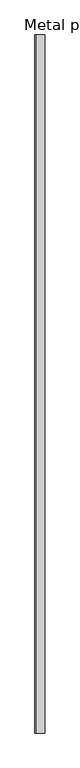
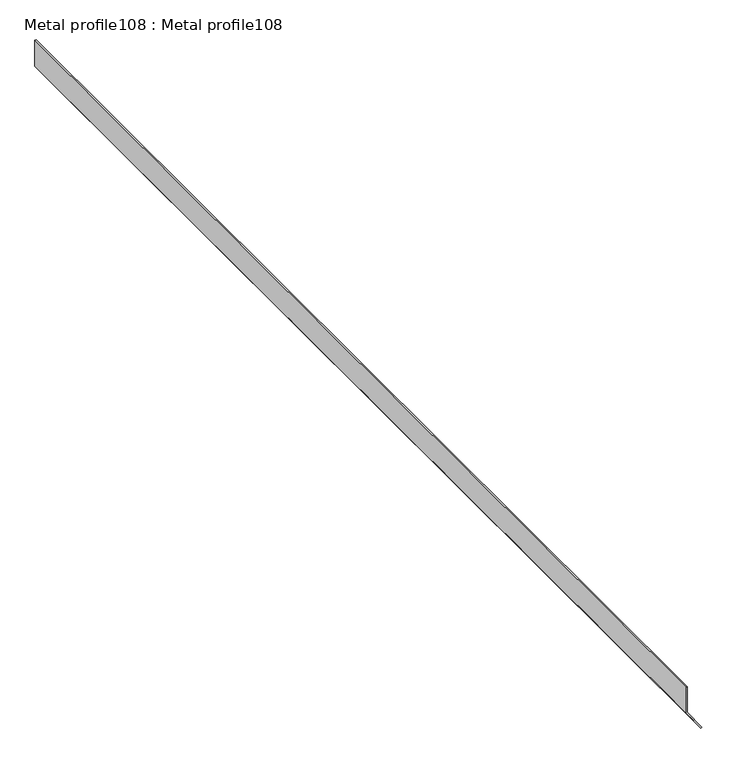
"""IFC4 building model written with IfcOpenShell, lengths in millimetres: proxy geometry, Metal profile108 : Metal profile108."""

from ifc_helpers import new_model, si_unit, frame, origin, place, context, project, spatial, polyline, outline, extrude, source, transform, mapped, element, save


def metal_profile108_metal_profile108_eef284db(model_context):
    return source(origin(), model_context, "Body", "SweptSolid", [
        extrude(outline(polyline([(41414.8071316, 6154.9411918), (41414.8071316, 6152.9411918), (41366.101002, 6152.9411918), (41328.7098067, 6179.0945686), (41329.8561294, 6180.7334537), (41366.7310426, 6154.9411918), (41414.8071316, 6154.9411918)])), frame((0.0, 2217.3609988, 0.0), z_axis=(0.0, 1.0, 0.0), x_axis=(0.0, 0.0, 1.0)), (0.0, 0.0, 1.0), 2000.0),
    ])


if __name__ == "__main__":
    model = new_model("IFC4")
    model_context = context("Model", 3, world=origin())
    ifc_project = project(units=[si_unit("LENGTHUNIT", "METRE", prefix="MILLI")], contexts=[model_context])
    site = spatial("IfcSite", under=ifc_project)
    building = spatial("IfcBuilding", under=site)
    placement = place(None, origin())
    metal_profile108_metal_profile108_shape = metal_profile108_metal_profile108_eef284db(model_context)
    element("IfcBuildingElementProxy", 1, Name="Metal profile108 : Metal profile108", ObjectType="Metal profile108 : Metal profile108", at=placement, inside=building, context=model_context, shape_type="MappedRepresentation", body=[
        mapped(metal_profile108_metal_profile108_shape, transform((0.0, 0.0, 0.0), x_axis=(1.0, 0.0, 0.0), y_axis=(0.0, 1.0, 0.0), z_axis=(0.0, 0.0, 1.0))),
    ])
    save(model, "model.ifc")

# Revit data of these elements
# Type "Metal profile108 : Metal profile108"
#   NameOverride = "Metal profile108"
# Element 1 (IfcBuildingElementProxy, "Metal profile108 : Metal profile108")
#   Materials on its faces: "TRIM CLEAT"
# Materials
#   "TRIM CLEAT": class "Unassigned", colour RGB 255 232 5, transparency 0
